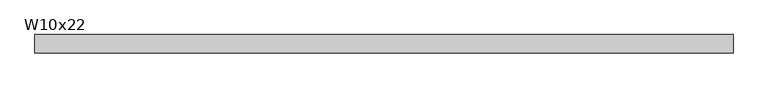
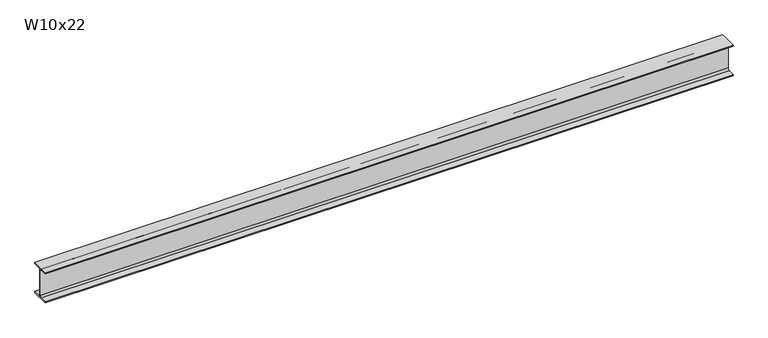
"""IFC4 building model written with IfcOpenShell, lengths in millimetres: beam geometry, RME W-Wide Flange : W10x22."""

import ifcopenshell
import ifcopenshell.guid

model = None  # the IFC model being written
_history = None  # IfcOwnerHistory: only IFC2X3 demands one
_inside = {}  # id of a spatial element -> (the spatial element, [elements in it])
_under = {}  # id of a project, library or spatial element -> (it, [spatial elements below it])
_declared = {}  # id of a project -> (the project, [libraries it declares])
_typed = {}  # id of a type object -> (the type object, [elements of that type])
_made_of = {}  # id of a material, layer set ... -> (it, [elements and type objects made of it])


def new_model(schema):
    """Start an empty IFC model of exactly this schema.

    Asked for "IFC4X3", IfcOpenShell would pick the latest addendum, in which some entities
    have other attributes; the version numbers below select the first issue.
    IFC2X3 requires an IfcOwnerHistory on every rooted entity: one is made here for all.
    """
    global model, _history
    if schema == "IFC4X3":
        model = ifcopenshell.file(schema_version=(4, 3, 0, 0))
    else:
        model = ifcopenshell.file(schema=schema)
    _inside.clear()
    _under.clear()
    _declared.clear()
    _typed.clear()
    _made_of.clear()
    _history = None
    if model.schema == "IFC2X3":
        org = make("IfcOrganization", Name="unknown")
        user = make(
            "IfcPersonAndOrganization",
            ThePerson=make("IfcPerson", FamilyName="unknown"),
            TheOrganization=org,
        )
        app = make(
            "IfcApplication",
            ApplicationDeveloper=org,
            Version="unknown",
            ApplicationFullName="unknown",
            ApplicationIdentifier="unknown",
        )
        _history = make(
            "IfcOwnerHistory",
            OwningUser=user,
            OwningApplication=app,
            ChangeAction="ADDED",
            CreationDate=0,
        )
    return model


def make(cls, **values):
    """One entity of the class cls with the attributes given. An attribute that is None is left unset."""
    return model.create_entity(
        cls, **{name: value for name, value in values.items() if value is not None}
    )


def rooted(cls, **values):
    """An entity with a GlobalId (a new one), such as an element, a storey or a relation."""
    return make(cls, GlobalId=ifcopenshell.guid.new(), OwnerHistory=_history, **values)


def si_unit(unit_type, name, prefix=None):
    """IfcSIUnit, for example si_unit("LENGTHUNIT", "METRE", prefix="MILLI")."""
    return make("IfcSIUnit", UnitType=unit_type, Prefix=prefix, Name=name)


def assignment(units):
    """IfcUnitAssignment: the units of a project."""
    return None if units is None else make("IfcUnitAssignment", Units=units)


def point(xyz):
    """IfcCartesianPoint."""
    return None if xyz is None else make("IfcCartesianPoint", Coordinates=xyz)


def direction(xyz):
    """IfcDirection."""
    return None if xyz is None else make("IfcDirection", DirectionRatios=xyz)


def frame(location, z_axis=None, x_axis=None):
    """IfcAxis2Placement3D, a coordinate frame: its origin and axes. An axis left out is left unset."""
    return make(
        "IfcAxis2Placement3D",
        Location=point(location),
        Axis=direction(z_axis),
        RefDirection=direction(x_axis),
    )


def frame_2d(location, x_axis=None):
    """IfcAxis2Placement2D, a coordinate frame in the plane: its origin and x axis."""
    return make(
        "IfcAxis2Placement2D", Location=point(location), RefDirection=direction(x_axis)
    )


def origin():
    """The frame at (0, 0, 0) with its axes left unset."""
    return frame((0.0, 0.0, 0.0))


def place(relative_to, where):
    """IfcLocalPlacement: puts the frame where relative to a parent placement (None: the world)."""
    return make(
        "IfcLocalPlacement", PlacementRelTo=relative_to, RelativePlacement=where
    )


def context(
    kind, dimensions, precision=None, world=None, true_north=None, identifier=None
):
    """IfcGeometricRepresentationContext, for example the 3D "Model" context."""
    return make(
        "IfcGeometricRepresentationContext",
        ContextIdentifier=identifier,
        ContextType=kind,
        CoordinateSpaceDimension=dimensions,
        Precision=precision,
        WorldCoordinateSystem=world,
        TrueNorth=true_north,
    )


def project(units=None, contexts=None):
    """IfcProject with its units and contexts."""
    return rooted(
        "IfcProject",
        Name="project",
        RepresentationContexts=contexts,
        UnitsInContext=assignment(units),
    )


def spatial(cls, under=None, at=None, **own):
    """A site, building, storey or space (cls), placed at a placement, below another one or the project."""
    s = rooted(cls, ObjectPlacement=at, **own)
    if under is not None:
        _under.setdefault(under.id(), (under, []))[1].append(s)
    return s


def polyline(points):
    """IfcPolyline through the points."""
    return make("IfcPolyline", Points=[point(p) for p in points])


def circle_curve(where, radius):
    """IfcCircle in the frame where."""
    return make("IfcCircle", Position=where, Radius=radius)


def trimmed(basis, trim1, trim2, sense, master):
    """IfcTrimmedCurve: the piece of a basis curve between two trims."""
    return make(
        "IfcTrimmedCurve",
        BasisCurve=basis,
        Trim1=trim1,
        Trim2=trim2,
        SenseAgreement=sense,
        MasterRepresentation=master,
    )


def segment(curve, same_sense, transition):
    """IfcCompositeCurveSegment."""
    return make(
        "IfcCompositeCurveSegment",
        Transition=transition,
        SameSense=same_sense,
        ParentCurve=curve,
    )


def composite_curve(segments, self_intersect=None):
    """IfcCompositeCurve: segments joined end to end."""
    return make("IfcCompositeCurve", Segments=segments, SelfIntersect=self_intersect)


def outline(outer, holes=None, kind="AREA"):
    """IfcArbitraryClosedProfileDef: a profile drawn as a closed curve; with holes, ...WithVoids."""
    if holes is None:
        return make("IfcArbitraryClosedProfileDef", ProfileType=kind, OuterCurve=outer)
    return make(
        "IfcArbitraryProfileDefWithVoids",
        ProfileType=kind,
        OuterCurve=outer,
        InnerCurves=holes,
    )


def extrude(swept, where, along, depth):
    """IfcExtrudedAreaSolid: the profile swept, set in the frame where, extruded along a direction by depth."""
    return make(
        "IfcExtrudedAreaSolid",
        SweptArea=swept,
        Position=where,
        ExtrudedDirection=direction(along),
        Depth=depth,
    )


def shape(context_of_items, identifier, shape_type, items):
    """IfcShapeRepresentation: the items that make up one representation, for example the "Body"."""
    return make(
        "IfcShapeRepresentation",
        ContextOfItems=context_of_items,
        RepresentationIdentifier=identifier,
        RepresentationType=shape_type,
        Items=items,
    )


def source(mapping_origin, context_of_items, identifier, shape_type, items):
    """IfcRepresentationMap: a shape defined once, which mapped items show again and again."""
    return make(
        "IfcRepresentationMap",
        MappingOrigin=mapping_origin,
        MappedRepresentation=shape(context_of_items, identifier, shape_type, items),
    )


def transform(
    local_origin,
    x_axis=None,
    y_axis=None,
    z_axis=None,
    scale=None,
    scale2=None,
    scale3=None,
    uniform=True,
):
    """IfcCartesianTransformationOperator3D, or its non-uniform kind. x_axis, y_axis, z_axis: its Axis1, 2, 3."""
    if uniform:
        return make(
            "IfcCartesianTransformationOperator3D",
            Axis1=direction(x_axis),
            Axis2=direction(y_axis),
            LocalOrigin=point(local_origin),
            Scale=scale,
            Axis3=direction(z_axis),
        )
    return make(
        "IfcCartesianTransformationOperator3DnonUniform",
        Axis1=direction(x_axis),
        Axis2=direction(y_axis),
        LocalOrigin=point(local_origin),
        Scale=scale,
        Axis3=direction(z_axis),
        Scale2=scale2,
        Scale3=scale3,
    )


def mapped(mapping_source, mapping_target):
    """IfcMappedItem: shows the shape of a source again, moved by a transform."""
    return make(
        "IfcMappedItem", MappingSource=mapping_source, MappingTarget=mapping_target
    )


def made_of(thing, what):
    """Note that an element or type object is made of a material, layer set ...; save() writes the relation."""
    if what is not None:
        _made_of.setdefault(what.id(), (what, []))[1].append(thing)
    return thing


def element(
    cls,
    number,
    at=None,
    inside=None,
    cuts=None,
    type_object=None,
    material=None,
    context=None,
    identifier="Body",
    shape_type=None,
    held_by="IfcProductDefinitionShape",
    body=None,
    shapes=None,
    **own,
):
    """One element of the class cls, such as IfcWall. Its Tag is "e" and its number.

    at: its placement. inside: the storey or other place that contains it. cuts: it is an
    opening in that element (IfcRelVoidsElement). A single representation is given by context,
    identifier, shape_type and body (its items); several are given by shapes. held_by: the class
    of the entity that holds the representations. save() writes the other relations.
    """
    e = rooted(cls, Tag="e%d" % number, ObjectPlacement=at, **own)
    if body is not None:
        shapes = [shape(context, identifier, shape_type, body)]
    if shapes is not None:
        e.Representation = make(held_by, Representations=shapes)
    if inside is not None:
        _inside.setdefault(inside.id(), (inside, []))[1].append(e)
    if cuts is not None:
        rooted(
            "IfcRelVoidsElement", RelatingBuildingElement=cuts, RelatedOpeningElement=e
        )
    if type_object is not None:
        _typed.setdefault(type_object.id(), (type_object, []))[1].append(e)
    return made_of(e, material)


def aggregate(whole, parts):
    """IfcRelAggregates: a whole, such as a stair, and the parts it consists of."""
    return rooted("IfcRelAggregates", RelatingObject=whole, RelatedObjects=parts)


def save(model, path):
    """Write the relations noted so far, then the file.

    IfcRelAggregates (storeys below a building ...), IfcRelContainedInSpatialStructure (elements
    in a storey), IfcRelDefinesByType, IfcRelAssociatesMaterial and IfcRelDeclares: one each for
    every whole, place, type object, material and project.
    """
    for whole, parts in _under.values():
        aggregate(whole, parts)
    for where, things in _inside.values():
        rooted(
            "IfcRelContainedInSpatialStructure",
            RelatedElements=things,
            RelatingStructure=where,
        )
    for kind, things in _typed.values():
        rooted("IfcRelDefinesByType", RelatedObjects=things, RelatingType=kind)
    for what, things in _made_of.values():
        rooted("IfcRelAssociatesMaterial", RelatedObjects=things, RelatingMaterial=what)
    for by, libraries in _declared.values():
        rooted("IfcRelDeclares", RelatingContext=by, RelatedDefinitions=libraries)
    model.write(path)


def w10x22_d9664158(model_context):
    return source(origin(), model_context, "Body", "SweptSolid", [
        extrude(outline(composite_curve([segment(polyline([(73.025, -120.396), (73.025, -129.54), (-73.025, -129.54), (-73.025, -120.396), (-17.7165, -120.396)]), True, "CONTINUOUS"), segment(trimmed(circle_curve(frame_2d((-17.7165, -105.7275)), 14.6685), [point((-17.7165, -120.396))], [point((-3.048, -105.7275))], True, "CARTESIAN"), True, "CONTINUOUS"), segment(polyline([(-3.048, -105.7275), (-3.048, 105.7275)]), True, "CONTINUOUS"), segment(trimmed(circle_curve(frame_2d((-17.7165, 105.7275)), 14.6685), [point((-3.048, 105.7275))], [point((-17.7165, 120.396))], True, "CARTESIAN"), True, "CONTINUOUS"), segment(polyline([(-17.7165, 120.396), (-73.025, 120.396), (-73.025, 129.54), (73.025, 129.54), (73.025, 120.396), (17.7165, 120.396)]), True, "CONTINUOUS"), segment(trimmed(circle_curve(frame_2d((17.7165, 105.7275)), 14.6685), [point((17.7165, 120.396))], [point((3.048, 105.7275))], True, "CARTESIAN"), True, "CONTINUOUS"), segment(polyline([(3.048, 105.7275), (3.048, -105.7275)]), True, "CONTINUOUS"), segment(trimmed(circle_curve(frame_2d((17.7165, -105.7275)), 14.6685), [point((3.048, -105.7275))], [point((17.7165, -120.396))], True, "CARTESIAN"), True, "CONTINUOUS"), segment(polyline([(17.7165, -120.396), (73.025, -120.396)]), True, "CONTINUOUS")], self_intersect=False)), frame((-2671.4739425, 0.0, 0.0), z_axis=(1.0, 0.0, 0.0), x_axis=(0.0, 1.0, 0.0)), (0.0, 0.0, 1.0), 5552.3749474),
    ])


if __name__ == "__main__":
    model = new_model("IFC4")
    model_context = context("Model", 3, world=origin())
    ifc_project = project(units=[si_unit("LENGTHUNIT", "METRE", prefix="MILLI")], contexts=[model_context])
    site = spatial("IfcSite", under=ifc_project)
    building = spatial("IfcBuilding", under=site)
    placement = place(None, origin())
    w10x22_shape = w10x22_d9664158(model_context)
    element("IfcBeam", 1, ObjectType="RME W-Wide Flange : W10x22", at=placement, inside=building, context=model_context, shape_type="MappedRepresentation", body=[
        mapped(w10x22_shape, transform((0.0, 0.0, 0.0), x_axis=(1.0, 0.0, 0.0), y_axis=(0.0, 1.0, 0.0), z_axis=(0.0, 0.0, 1.0))),
    ])
    save(model, "model.ifc")

# Revit data of these elements
# Type "RME W-Wide Flange : W10x22"
#   WELD P [instance default] = ""
#   WELD LE [instance default] = ""
#   WELD D [instance default] = ""
#   TOP SECTION SIZE [instance default] = ""
#   TOP SECTION LENGTH [instance default] = ""
#   REMARKS [instance default] = ""
#   REINF TYPE [instance default] = ""
#   Nominal Size = "W24"
#   End Bearing Capacity [instance default] = ""
#   BOT SECTION SIZE [instance default] = ""
#   BOT SECTION LENGTH [instance default] = ""
#   Assembly Code = "B10"
#   W = 22
#   Start Extension Calculation [instance default] = 10' - 0"
#   Start Extension [instance default] = -0' - 0 1/2"
#   End Extension Calculation [instance default] = 10' - 0"
#   End Extension [instance default] = -0' - 0 1/2"
#   Length [instance default] = 5' - 0"
#   bf = 0' - 5 3/4"
#   d = 0' - 10.2"
#   k = 0' - 0 15/16"
#   k2 = 0' - 0.5775"
#   tf = 0' - 0.36"
#   tw = 0' - 0.24"
#   A = 0.0450694 SF
#   Structural Material [instance default] = Metal - Steel - ASTM A992
# Element 1 (IfcBeam, "RME W-Wide Flange : W10x22")
#   End Extension Calculation = 10' - 3.4213"
#   End Extension = 0' - 2.9213"
#   Length = 18' - 4"
#   Materials on its faces: "Metal - Steel - ASTM A992"
# Materials
#   "Metal - Steel - ASTM A992": class "Metal", colour RGB 255 128 0, transparency 0
